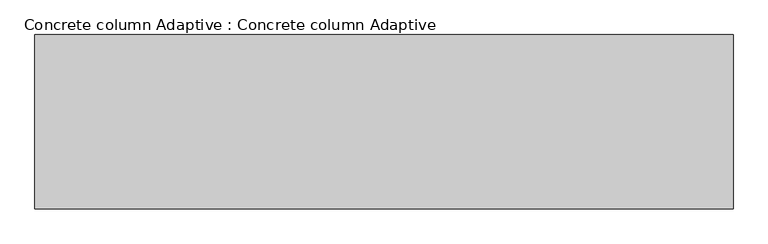
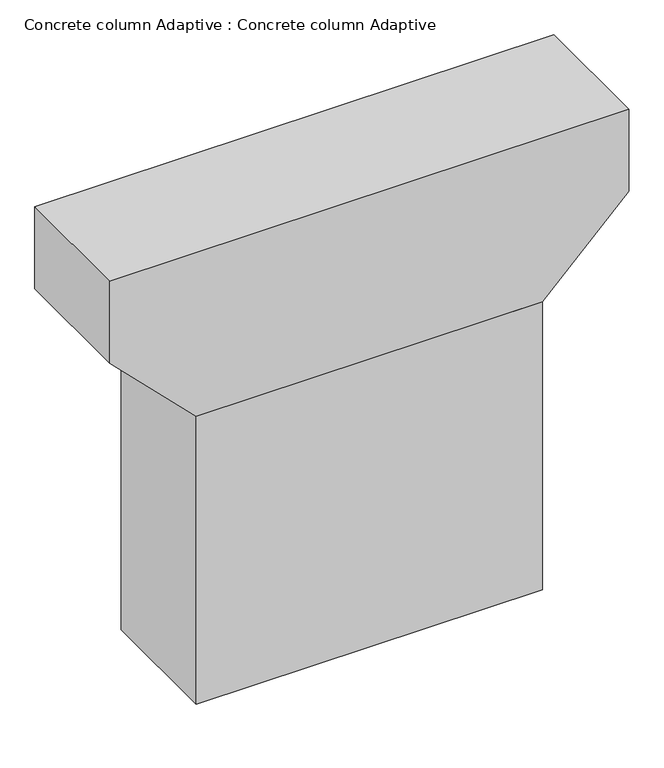
"""IFC4 building model written with IfcOpenShell, lengths in millimetres: proxy geometry, Concrete column Adaptive : Concrete column Adaptive."""

from ifc_helpers import new_model, si_unit, frame, origin, origin_with_axes, place, context, project, spatial, polyline, outline, extrude, source, transform, mapped, element, save


def concrete_column_adaptive_concrete_column_adaptive_77980e97(model_context):
    return source(origin(), model_context, "Body", "SweptSolid", [
        extrude(outline(polyline([(11034.0, 6000.0), (11034.0, -6000.0), (9034.0, -6000.0), (7034.0, -4000.0), (7034.0, 4000.0), (9034.0, 6000.0), (11034.0, 6000.0)])), frame((0.0, -1500.0, 0.0), z_axis=(0.0, 1.0, 0.0), x_axis=(0.0, 0.0, 1.0)), (0.0, 0.0, 1.0), 3000.0),
        extrude(outline(polyline([(-4000.0, -1500.0), (-4000.0, 1500.0), (4000.0, 1500.0), (4000.0, -1500.0), (-4000.0, -1500.0)])), origin_with_axes(), (0.0, 0.0, 1.0), 7034.0),
    ])


if __name__ == "__main__":
    model = new_model("IFC4")
    model_context = context("Model", 3, world=origin())
    ifc_project = project(units=[si_unit("LENGTHUNIT", "METRE", prefix="MILLI")], contexts=[model_context])
    site = spatial("IfcSite", under=ifc_project)
    building = spatial("IfcBuilding", under=site)
    placement = place(None, origin())
    concrete_column_adaptive_concrete_column_adaptive_shape = concrete_column_adaptive_concrete_column_adaptive_77980e97(model_context)
    element("IfcBuildingElementProxy", 1, Name="Concrete column Adaptive : Concrete column Adaptive", ObjectType="Concrete column Adaptive : Concrete column Adaptive", at=placement, inside=building, context=model_context, shape_type="MappedRepresentation", body=[
        mapped(concrete_column_adaptive_concrete_column_adaptive_shape, transform((0.0, 0.0, 0.0), x_axis=(1.0, 0.0, 0.0), y_axis=(0.0, 1.0, 0.0), z_axis=(0.0, 0.0, 1.0))),
    ])
    save(model, "model.ifc")

# Revit data of these elements
# Type "Concrete column Adaptive : Concrete column Adaptive"
#   Height [instance default] = 30000 mm
#   Default Elevation = 0
# Element 1 (IfcBuildingElementProxy, "Concrete column Adaptive : Concrete column Adaptive")
#   Height = 7034 mm
#   Materials on its faces: "Default Wall"
# Materials
#   "Default Wall": class "Miscellaneous", colour RGB 128 128 128, transparency 0, Comments = "Rendering appearance not upgraded Rendering appearance not upgraded ", Cost = 0
